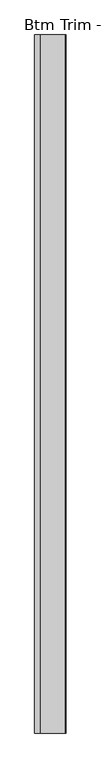
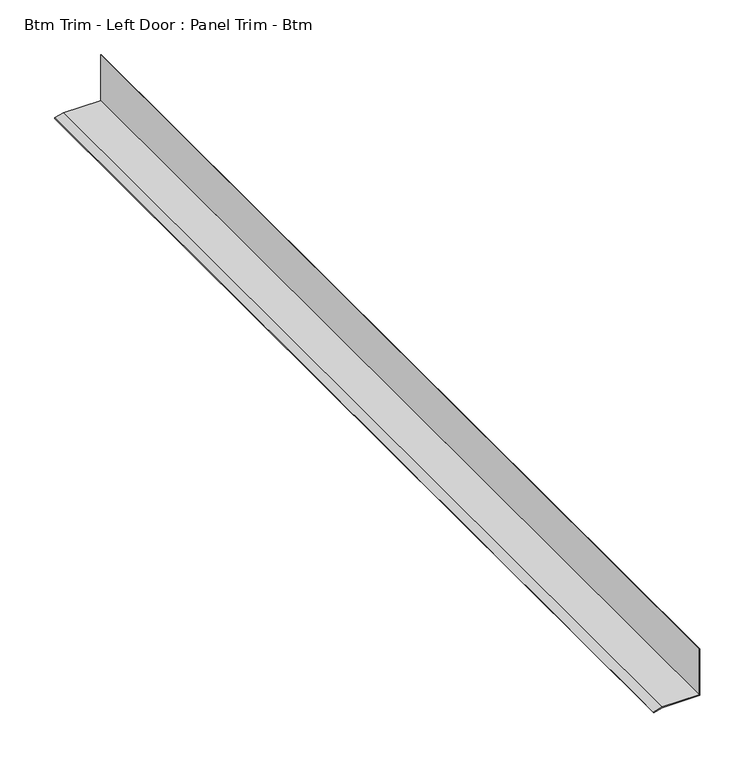
"""IFC4 building model written with IfcOpenShell, lengths in millimetres: proxy geometry, Btm Trim - Left Door : Panel Trim - Btm."""

import ifcopenshell
import ifcopenshell.guid

model = None  # the IFC model being written
_history = None  # IfcOwnerHistory: only IFC2X3 demands one
_inside = {}  # id of a spatial element -> (the spatial element, [elements in it])
_under = {}  # id of a project, library or spatial element -> (it, [spatial elements below it])
_declared = {}  # id of a project -> (the project, [libraries it declares])
_typed = {}  # id of a type object -> (the type object, [elements of that type])
_made_of = {}  # id of a material, layer set ... -> (it, [elements and type objects made of it])


def new_model(schema):
    """Start an empty IFC model of exactly this schema.

    Asked for "IFC4X3", IfcOpenShell would pick the latest addendum, in which some entities
    have other attributes; the version numbers below select the first issue.
    IFC2X3 requires an IfcOwnerHistory on every rooted entity: one is made here for all.
    """
    global model, _history
    if schema == "IFC4X3":
        model = ifcopenshell.file(schema_version=(4, 3, 0, 0))
    else:
        model = ifcopenshell.file(schema=schema)
    _inside.clear()
    _under.clear()
    _declared.clear()
    _typed.clear()
    _made_of.clear()
    _history = None
    if model.schema == "IFC2X3":
        org = make("IfcOrganization", Name="unknown")
        user = make(
            "IfcPersonAndOrganization",
            ThePerson=make("IfcPerson", FamilyName="unknown"),
            TheOrganization=org,
        )
        app = make(
            "IfcApplication",
            ApplicationDeveloper=org,
            Version="unknown",
            ApplicationFullName="unknown",
            ApplicationIdentifier="unknown",
        )
        _history = make(
            "IfcOwnerHistory",
            OwningUser=user,
            OwningApplication=app,
            ChangeAction="ADDED",
            CreationDate=0,
        )
    return model


def make(cls, **values):
    """One entity of the class cls with the attributes given. An attribute that is None is left unset."""
    return model.create_entity(
        cls, **{name: value for name, value in values.items() if value is not None}
    )


def rooted(cls, **values):
    """An entity with a GlobalId (a new one), such as an element, a storey or a relation."""
    return make(cls, GlobalId=ifcopenshell.guid.new(), OwnerHistory=_history, **values)


def si_unit(unit_type, name, prefix=None):
    """IfcSIUnit, for example si_unit("LENGTHUNIT", "METRE", prefix="MILLI")."""
    return make("IfcSIUnit", UnitType=unit_type, Prefix=prefix, Name=name)


def assignment(units):
    """IfcUnitAssignment: the units of a project."""
    return None if units is None else make("IfcUnitAssignment", Units=units)


def point(xyz):
    """IfcCartesianPoint."""
    return None if xyz is None else make("IfcCartesianPoint", Coordinates=xyz)


def direction(xyz):
    """IfcDirection."""
    return None if xyz is None else make("IfcDirection", DirectionRatios=xyz)


def frame(location, z_axis=None, x_axis=None):
    """IfcAxis2Placement3D, a coordinate frame: its origin and axes. An axis left out is left unset."""
    return make(
        "IfcAxis2Placement3D",
        Location=point(location),
        Axis=direction(z_axis),
        RefDirection=direction(x_axis),
    )


def origin():
    """The frame at (0, 0, 0) with its axes left unset."""
    return frame((0.0, 0.0, 0.0))


def place(relative_to, where):
    """IfcLocalPlacement: puts the frame where relative to a parent placement (None: the world)."""
    return make(
        "IfcLocalPlacement", PlacementRelTo=relative_to, RelativePlacement=where
    )


def context(
    kind, dimensions, precision=None, world=None, true_north=None, identifier=None
):
    """IfcGeometricRepresentationContext, for example the 3D "Model" context."""
    return make(
        "IfcGeometricRepresentationContext",
        ContextIdentifier=identifier,
        ContextType=kind,
        CoordinateSpaceDimension=dimensions,
        Precision=precision,
        WorldCoordinateSystem=world,
        TrueNorth=true_north,
    )


def project(units=None, contexts=None):
    """IfcProject with its units and contexts."""
    return rooted(
        "IfcProject",
        Name="project",
        RepresentationContexts=contexts,
        UnitsInContext=assignment(units),
    )


def spatial(cls, under=None, at=None, **own):
    """A site, building, storey or space (cls), placed at a placement, below another one or the project."""
    s = rooted(cls, ObjectPlacement=at, **own)
    if under is not None:
        _under.setdefault(under.id(), (under, []))[1].append(s)
    return s


def polyline(points):
    """IfcPolyline through the points."""
    return make("IfcPolyline", Points=[point(p) for p in points])


def outline(outer, holes=None, kind="AREA"):
    """IfcArbitraryClosedProfileDef: a profile drawn as a closed curve; with holes, ...WithVoids."""
    if holes is None:
        return make("IfcArbitraryClosedProfileDef", ProfileType=kind, OuterCurve=outer)
    return make(
        "IfcArbitraryProfileDefWithVoids",
        ProfileType=kind,
        OuterCurve=outer,
        InnerCurves=holes,
    )


def extrude(swept, where, along, depth):
    """IfcExtrudedAreaSolid: the profile swept, set in the frame where, extruded along a direction by depth."""
    return make(
        "IfcExtrudedAreaSolid",
        SweptArea=swept,
        Position=where,
        ExtrudedDirection=direction(along),
        Depth=depth,
    )


def shape(context_of_items, identifier, shape_type, items):
    """IfcShapeRepresentation: the items that make up one representation, for example the "Body"."""
    return make(
        "IfcShapeRepresentation",
        ContextOfItems=context_of_items,
        RepresentationIdentifier=identifier,
        RepresentationType=shape_type,
        Items=items,
    )


def source(mapping_origin, context_of_items, identifier, shape_type, items):
    """IfcRepresentationMap: a shape defined once, which mapped items show again and again."""
    return make(
        "IfcRepresentationMap",
        MappingOrigin=mapping_origin,
        MappedRepresentation=shape(context_of_items, identifier, shape_type, items),
    )


def transform(
    local_origin,
    x_axis=None,
    y_axis=None,
    z_axis=None,
    scale=None,
    scale2=None,
    scale3=None,
    uniform=True,
):
    """IfcCartesianTransformationOperator3D, or its non-uniform kind. x_axis, y_axis, z_axis: its Axis1, 2, 3."""
    if uniform:
        return make(
            "IfcCartesianTransformationOperator3D",
            Axis1=direction(x_axis),
            Axis2=direction(y_axis),
            LocalOrigin=point(local_origin),
            Scale=scale,
            Axis3=direction(z_axis),
        )
    return make(
        "IfcCartesianTransformationOperator3DnonUniform",
        Axis1=direction(x_axis),
        Axis2=direction(y_axis),
        LocalOrigin=point(local_origin),
        Scale=scale,
        Axis3=direction(z_axis),
        Scale2=scale2,
        Scale3=scale3,
    )


def mapped(mapping_source, mapping_target):
    """IfcMappedItem: shows the shape of a source again, moved by a transform."""
    return make(
        "IfcMappedItem", MappingSource=mapping_source, MappingTarget=mapping_target
    )


def made_of(thing, what):
    """Note that an element or type object is made of a material, layer set ...; save() writes the relation."""
    if what is not None:
        _made_of.setdefault(what.id(), (what, []))[1].append(thing)
    return thing


def element(
    cls,
    number,
    at=None,
    inside=None,
    cuts=None,
    type_object=None,
    material=None,
    context=None,
    identifier="Body",
    shape_type=None,
    held_by="IfcProductDefinitionShape",
    body=None,
    shapes=None,
    **own,
):
    """One element of the class cls, such as IfcWall. Its Tag is "e" and its number.

    at: its placement. inside: the storey or other place that contains it. cuts: it is an
    opening in that element (IfcRelVoidsElement). A single representation is given by context,
    identifier, shape_type and body (its items); several are given by shapes. held_by: the class
    of the entity that holds the representations. save() writes the other relations.
    """
    e = rooted(cls, Tag="e%d" % number, ObjectPlacement=at, **own)
    if body is not None:
        shapes = [shape(context, identifier, shape_type, body)]
    if shapes is not None:
        e.Representation = make(held_by, Representations=shapes)
    if inside is not None:
        _inside.setdefault(inside.id(), (inside, []))[1].append(e)
    if cuts is not None:
        rooted(
            "IfcRelVoidsElement", RelatingBuildingElement=cuts, RelatedOpeningElement=e
        )
    if type_object is not None:
        _typed.setdefault(type_object.id(), (type_object, []))[1].append(e)
    return made_of(e, material)


def aggregate(whole, parts):
    """IfcRelAggregates: a whole, such as a stair, and the parts it consists of."""
    return rooted("IfcRelAggregates", RelatingObject=whole, RelatedObjects=parts)


def save(model, path):
    """Write the relations noted so far, then the file.

    IfcRelAggregates (storeys below a building ...), IfcRelContainedInSpatialStructure (elements
    in a storey), IfcRelDefinesByType, IfcRelAssociatesMaterial and IfcRelDeclares: one each for
    every whole, place, type object, material and project.
    """
    for whole, parts in _under.values():
        aggregate(whole, parts)
    for where, things in _inside.values():
        rooted(
            "IfcRelContainedInSpatialStructure",
            RelatedElements=things,
            RelatingStructure=where,
        )
    for kind, things in _typed.values():
        rooted("IfcRelDefinesByType", RelatedObjects=things, RelatingType=kind)
    for what, things in _made_of.values():
        rooted("IfcRelAssociatesMaterial", RelatedObjects=things, RelatingMaterial=what)
    for by, libraries in _declared.values():
        rooted("IfcRelDeclares", RelatingContext=by, RelatedDefinitions=libraries)
    model.write(path)


def btm_trim_left_door_panel_trim_btm_813b1cb6(model_context):
    return source(origin(), model_context, "Body", "SweptSolid", [
        extrude(outline(polyline([(50.8, 587326.1141748), (48.3077022, 587316.8127928), (47.5409986, 587317.0182304), (50.00625, 587326.2186739), (50.00625, 587365.8934739), (101.6, 587365.8934739), (101.6, 587365.1060739), (50.8, 587365.1060739), (50.8, 587326.1141748)])), frame((0.0, -532878.2537841, 0.0), z_axis=(0.0, 1.0, 0.0), x_axis=(0.0, 0.0, 1.0)), (0.0, 0.0, 1.0), 1093.7880247),
    ])


if __name__ == "__main__":
    model = new_model("IFC4")
    model_context = context("Model", 3, world=origin())
    ifc_project = project(units=[si_unit("LENGTHUNIT", "METRE", prefix="MILLI")], contexts=[model_context])
    site = spatial("IfcSite", under=ifc_project)
    building = spatial("IfcBuilding", under=site)
    placement = place(None, origin())
    btm_trim_left_door_panel_trim_btm_shape = btm_trim_left_door_panel_trim_btm_813b1cb6(model_context)
    element("IfcBuildingElementProxy", 1, Name="Btm Trim - Left Door : Panel Trim - Btm", ObjectType="Btm Trim - Left Door : Panel Trim - Btm", at=placement, inside=building, context=model_context, shape_type="MappedRepresentation", body=[
        mapped(btm_trim_left_door_panel_trim_btm_shape, transform((0.0, 0.0, 0.0), x_axis=(1.0, 0.0, 0.0), y_axis=(0.0, 1.0, 0.0), z_axis=(0.0, 0.0, 1.0))),
    ])
    save(model, "model.ifc")

# Revit data of these elements
# Element 1 (IfcBuildingElementProxy, "Btm Trim - Left Door : Panel Trim - Btm")
#   Materials on its faces: "BASE TRIM BY MTL PANEL MFR."
# Materials
#   "BASE TRIM BY MTL PANEL MFR.": class "Generic", colour RGB 239 242 240, transparency 0, Cost = 0
